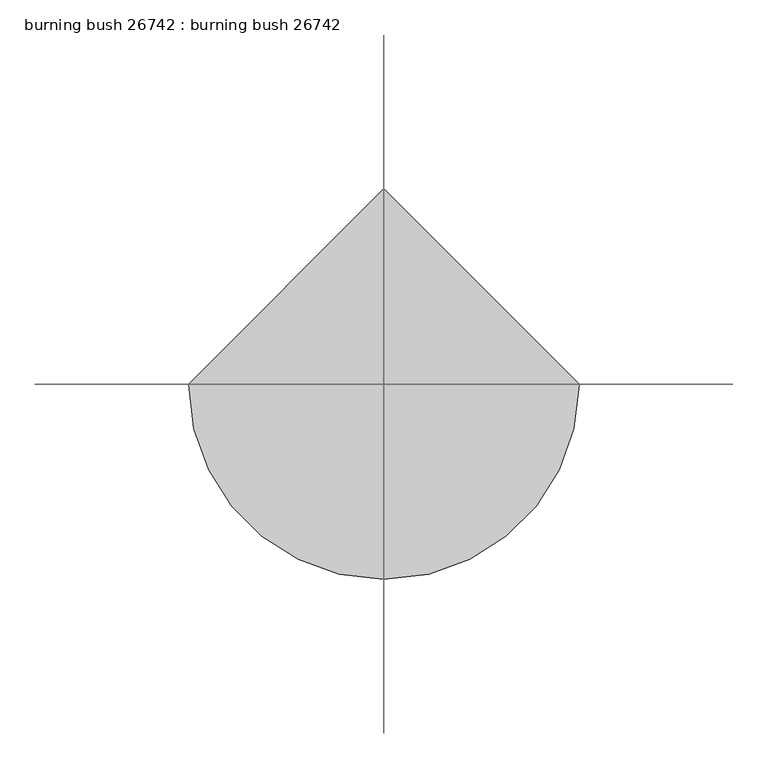
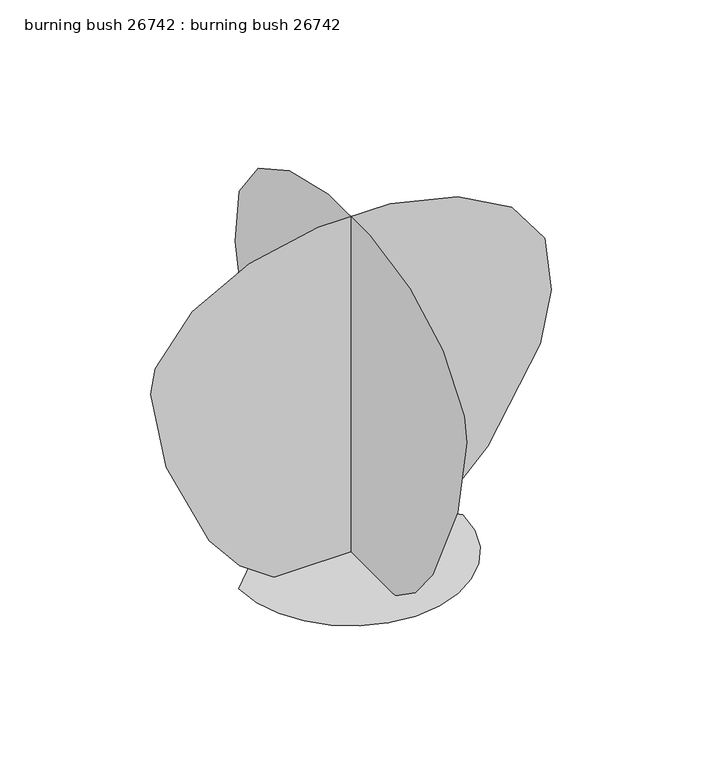
"""IFC4 building model written with IfcOpenShell, lengths in millimetres: proxy geometry, burning bush 26742 : burning bush 26742."""

from ifc_helpers import new_model, si_unit, origin, place, context, project, spatial, triangles, source, transform, mapped, element, save


def burning_bush_26742_burning_bush_26742_ca6e1e19(model_context):
    return source(origin(), model_context, "Body", "Tessellation", [
        triangles([(-433.0060553, 0.0, 9.6e-06), (-421.5583165, -99.2161097, 9.6e-06), (-388.9574358, -190.3303883, 9.6e-06), (-337.809504, -270.7307133, 9.6e-06), (-270.7307133, -337.809504, 9.6e-06), (-190.3301339, -388.9574358, 9.6e-06), (-99.2161097, -421.5583165, 9.6e-06), (1.89e-05, -433.0060553, 9.6e-06), (99.2161097, -421.5583165, 9.6e-06), (190.3303883, -388.9574358, 9.6e-06), (270.7307133, -337.809504, 9.6e-06), (337.8120475, -270.7307133, 9.6e-06), (388.9574358, -190.3301339, 9.6e-06), (421.5583165, -99.2161097, 9.6e-06), (433.0060553, 3.79e-05, 9.6e-06), (-5.68e-05, 433.0060553, 9.6e-06), (0.0014009, -430.765785, 94.2524501), (0.0014009, -546.9046263, 237.6063543), (0.0014009, -714.237145, 595.0121913), (0.0014009, -774.5366621, 915.4404888), (0.0014009, -756.8862133, 1012.5699526), (0.0014009, -613.7091242, 1195.6605938), (0.0014009, -392.9985772, 1314.6594349), (0.0014009, -126.9008115, 1371.5986919), (0.0014009, 152.4422576, 1368.5125431), (0.0014009, 412.8816659, 1307.4357479), (0.0014009, 622.2765518, 1190.4028479), (0.0014009, 748.478805, 1019.4483118), (0.0014009, 774.5341187, 800.0204264), (0.0014009, 730.9985493, 593.4373964), (0.0014009, 528.3042355, 247.0045997), (0.0014009, 284.5635354, 0.0), (0.0014009, -297.0654067, 0.7142016), (-430.7632416, -0.0013164, 94.2524501), (-546.9020828, -0.001325, 237.6063543), (-714.2346016, -0.0013463, 595.0121913), (-774.5341187, -0.0013654, 915.4404888), (-756.8836699, -0.0013711, 1012.5699526), (-613.7065807, -0.0013821, 1195.6605938), (-392.9960338, -0.0013892, 1314.6594349), (-126.8977685, -0.0013925, 1371.5986919), (152.4450554, -0.0013924, 1368.5125431), (412.8867528, -0.0013887, 1307.4357479), (622.2790226, -0.0013817, 1190.4028479), (748.4813484, -0.0013716, 1019.4483118), (774.5366621, -0.0013585, 800.0204264), (731.0010927, -0.0013462, 593.4373964), (528.3067789, -0.0013255, 247.0045997), (284.5660788, -0.0013108, 6.01e-05), (-297.0628633, -0.0013108, 0.7142625)], [[15, 16, 1], [14, 15, 1], [14, 1, 2], [13, 14, 2], [13, 2, 3], [13, 3, 4], [12, 13, 4], [11, 12, 4], [11, 4, 5], [11, 5, 6], [11, 6, 7], [11, 7, 8], [11, 8, 9], [11, 9, 10], [32, 33, 17], [32, 17, 18], [31, 32, 18], [31, 18, 19], [30, 31, 19], [29, 30, 19], [28, 29, 19], [27, 28, 19], [26, 27, 19], [25, 26, 19], [24, 25, 19], [23, 24, 19], [22, 23, 19], [21, 22, 19], [21, 19, 20], [49, 50, 34], [49, 34, 35], [48, 49, 35], [48, 35, 36], [47, 48, 36], [46, 47, 36], [45, 46, 36], [44, 45, 36], [43, 44, 36], [42, 43, 36], [41, 42, 36], [40, 41, 36], [39, 40, 36], [38, 39, 36], [38, 36, 37]], closed=False),
    ])


if __name__ == "__main__":
    model = new_model("IFC4")
    model_context = context("Model", 3, world=origin())
    ifc_project = project(units=[si_unit("LENGTHUNIT", "METRE", prefix="MILLI")], contexts=[model_context])
    site = spatial("IfcSite", under=ifc_project)
    building = spatial("IfcBuilding", under=site)
    placement = place(None, origin())
    burning_bush_26742_burning_bush_26742_shape = burning_bush_26742_burning_bush_26742_ca6e1e19(model_context)
    element("IfcBuildingElementProxy", 1, Name="burning bush 26742 : burning bush 26742", ObjectType="burning bush 26742 : burning bush 26742", at=placement, inside=building, context=model_context, shape_type="MappedRepresentation", body=[
        mapped(burning_bush_26742_burning_bush_26742_shape, transform((0.0, 0.0, 0.0), x_axis=(1.0, 0.0, 0.0), y_axis=(0.0, 1.0, 0.0), z_axis=(0.0, 0.0, 1.0))),
    ])
    save(model, "model.ifc")

# Revit data of these elements
# Type "burning bush 26742 : burning bush 26742"
#   built-in parameter 1005195 = "RPC-16-FVGW-0UXX-7JA7-N000-ST1L-LVER-AU"
#   Height = 0
